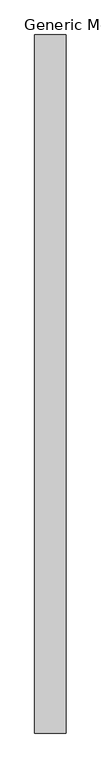
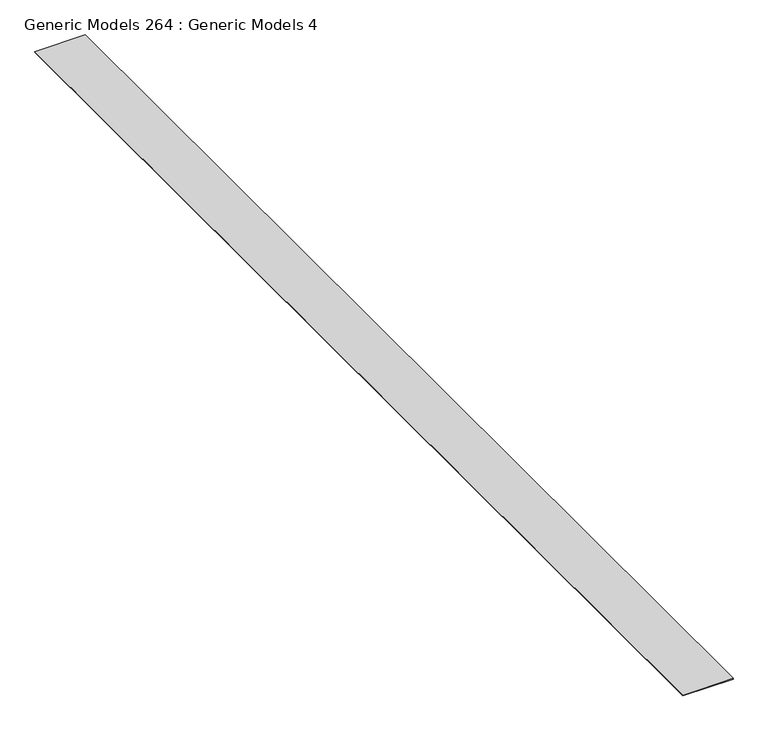
"""IFC4 building model written with IfcOpenShell, lengths in millimetres: proxy geometry, Generic Models 264 : Generic Models 4."""

from ifc_helpers import new_model, si_unit, frame, origin, place, context, project, spatial, polyline, outline, extrude, source, transform, mapped, element, save


def generic_models_264_generic_models_4_2d525cdd(model_context):
    return source(origin(), model_context, "Body", "SweptSolid", [
        extrude(outline(polyline([(1515.5714201, -5493.3230338), (949.9377059, -5493.3230338), (949.9377059, 7054.2769662), (1515.5714201, 7054.2769662), (1515.5714201, -5493.3230338)])), frame((0.0, 0.0, 123440.571), z_axis=(0.0, 0.0, 1.0), x_axis=(1.0, 0.0, 0.0)), (0.0, 0.0, 1.0), 9.525),
    ])


if __name__ == "__main__":
    model = new_model("IFC4")
    model_context = context("Model", 3, world=origin())
    ifc_project = project(units=[si_unit("LENGTHUNIT", "METRE", prefix="MILLI")], contexts=[model_context])
    site = spatial("IfcSite", under=ifc_project)
    building = spatial("IfcBuilding", under=site)
    placement = place(None, origin())
    generic_models_264_generic_models_4_shape = generic_models_264_generic_models_4_2d525cdd(model_context)
    element("IfcBuildingElementProxy", 1, Name="Generic Models 264 : Generic Models 4", ObjectType="Generic Models 264 : Generic Models 4", at=placement, inside=building, context=model_context, shape_type="MappedRepresentation", body=[
        mapped(generic_models_264_generic_models_4_shape, transform((0.0, 0.0, 0.0), x_axis=(1.0, 0.0, 0.0), y_axis=(0.0, 1.0, 0.0), z_axis=(0.0, 0.0, 1.0))),
    ])
    save(model, "model.ifc")

# Revit data of these elements
# Element 1 (IfcBuildingElementProxy, "Generic Models 264 : Generic Models 4")
#   Materials on its faces: "_CERAMIC TILE OR STONE FLOOR T.B.D."
# Materials
#   "_CERAMIC TILE OR STONE FLOOR T.B.D.": class "Generic", colour RGB 233 233 233, transparency 0, Cost = 0
